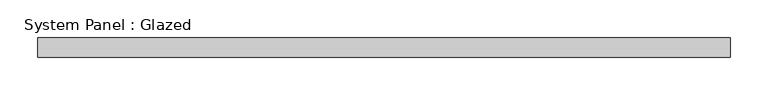
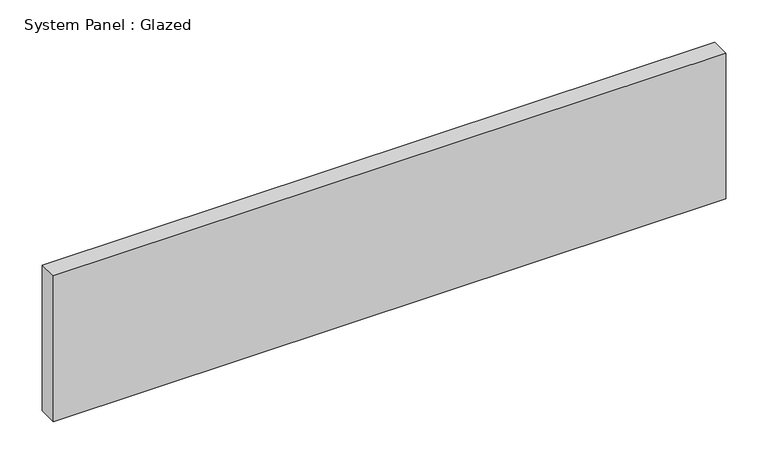
"""IFC4 building model written with IfcOpenShell, lengths in millimetres: plate geometry, System Panel : Glazed."""

from ifc_helpers import new_model, si_unit, origin, origin_with_axes, place, context, project, spatial, polyline, outline, extrude, source, transform, mapped, element, save


def system_panel_glazed_8dc8626f(model_context):
    return source(origin(), model_context, "Body", "SweptSolid", [
        extrude(outline(polyline([(457.2, -44.45), (-457.2, -44.45), (-457.2, -19.05), (457.2, -19.05), (457.2, -44.45)])), origin_with_axes(), (0.0, 0.0, 1.0), 209.55),
    ])


if __name__ == "__main__":
    model = new_model("IFC4")
    model_context = context("Model", 3, world=origin())
    ifc_project = project(units=[si_unit("LENGTHUNIT", "METRE", prefix="MILLI")], contexts=[model_context])
    site = spatial("IfcSite", under=ifc_project)
    building = spatial("IfcBuilding", under=site)
    placement = place(None, origin())
    system_panel_glazed_shape = system_panel_glazed_8dc8626f(model_context)
    element("IfcPlate", 1, ObjectType="System Panel : Glazed", at=placement, inside=building, context=model_context, shape_type="MappedRepresentation", body=[
        mapped(system_panel_glazed_shape, transform((0.0, 0.0, 0.0), x_axis=(1.0, 0.0, 0.0), y_axis=(0.0, 1.0, 0.0), z_axis=(0.0, 0.0, 1.0))),
    ])
    save(model, "model.ifc")

# Revit data of these elements
# Element 1 (IfcPlate, "System Panel : Glazed")
#   Materials on its faces: "Glass"
# Materials
#   "Glass": class "Glass", colour RGB 0 128 192, transparency 0.75
